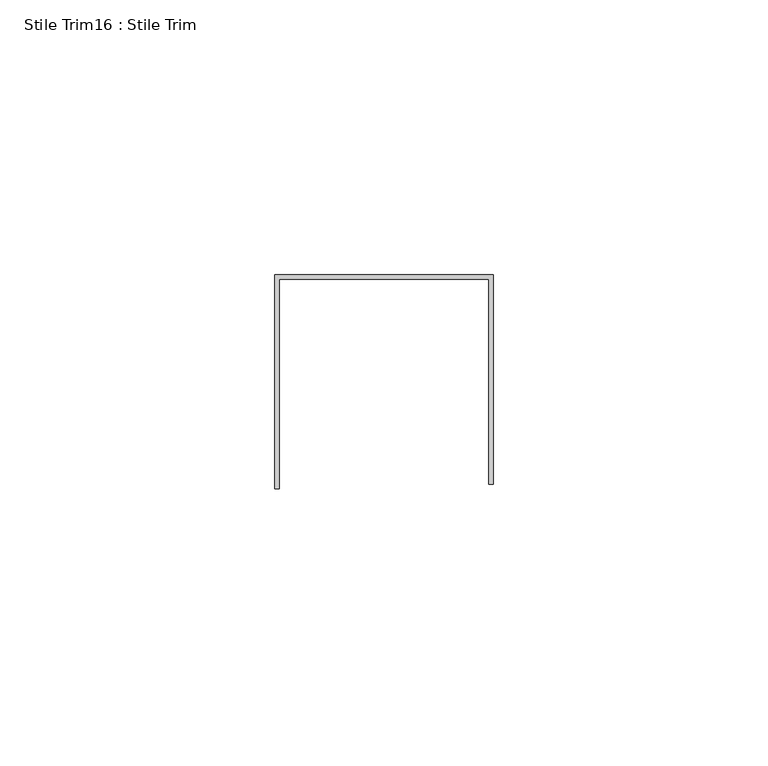
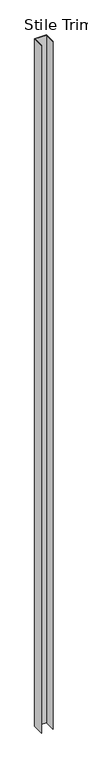
"""IFC4 building model written with IfcOpenShell, lengths in millimetres: proxy geometry, Stile Trim16 : Stile Trim."""

from ifc_helpers import new_model, si_unit, frame, origin, place, context, project, spatial, polyline, outline, extrude, source, transform, mapped, element, save


def stile_trim16_stile_trim_015bedb9(model_context):
    return source(origin(), model_context, "Body", "SweptSolid", [
        extrude(outline(polyline([(587327.0060739, -533994.2789841), (587366.6808739, -533994.2789841), (587366.6808739, -534032.3789841), (587365.8934739, -534032.3789841), (587365.8934739, -533995.0663841), (587327.7934739, -533995.0663841), (587327.7934739, -534033.1663841), (587327.0060739, -534033.1663841), (587327.0060739, -533994.2789841)])), frame((0.0, 0.0, 12.7), z_axis=(0.0, 0.0, 1.0), x_axis=(1.0, 0.0, 0.0)), (0.0, 0.0, 1.0), 2425.7),
    ])


if __name__ == "__main__":
    model = new_model("IFC4")
    model_context = context("Model", 3, world=origin())
    ifc_project = project(units=[si_unit("LENGTHUNIT", "METRE", prefix="MILLI")], contexts=[model_context])
    site = spatial("IfcSite", under=ifc_project)
    building = spatial("IfcBuilding", under=site)
    placement = place(None, origin())
    stile_trim16_stile_trim_shape = stile_trim16_stile_trim_015bedb9(model_context)
    element("IfcBuildingElementProxy", 1, Name="Stile Trim16 : Stile Trim", ObjectType="Stile Trim16 : Stile Trim", at=placement, inside=building, context=model_context, shape_type="MappedRepresentation", body=[
        mapped(stile_trim16_stile_trim_shape, transform((0.0, 0.0, 0.0), x_axis=(1.0, 0.0, 0.0), y_axis=(0.0, 1.0, 0.0), z_axis=(0.0, 0.0, 1.0))),
    ])
    save(model, "model.ifc")

# Revit data of these elements
# Project information
#   Project Issue Date = "Issue Date"
#   Project Status = "Project Status"
#   Client Name = "Xcel"
#   Project Address = "Enter address here"
#   Project Name = "Sports Complex"
#   Project Number = "Project Number"
# Element 1 (IfcBuildingElementProxy, "Stile Trim16 : Stile Trim")
#   Materials on its faces: "EDGE TRIM BY MTL PANEL MFR."
# Materials
#   "EDGE TRIM BY MTL PANEL MFR.": class "Generic", colour RGB 239 242 240, transparency 0, Cost = 0
